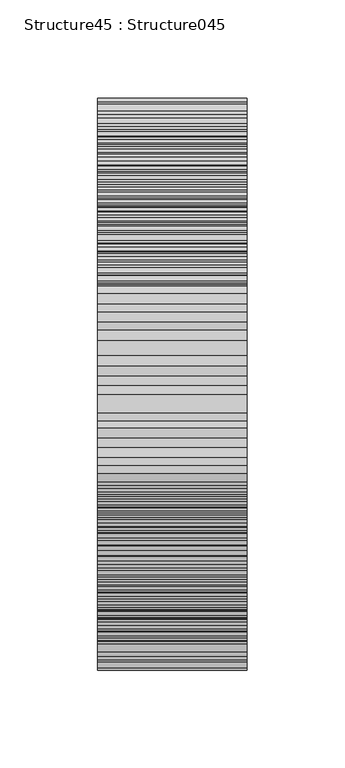
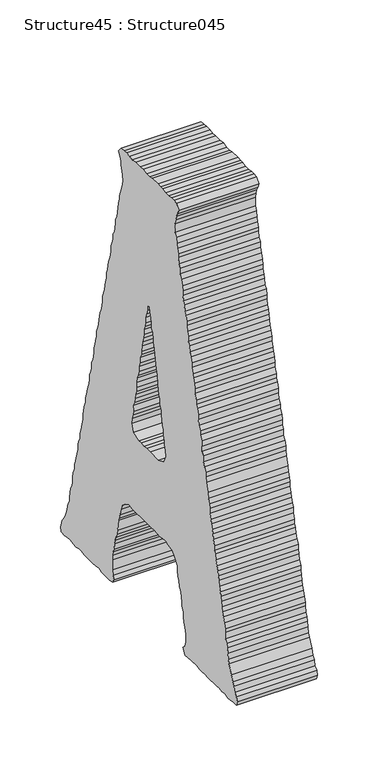
"""IFC4 building model written with IfcOpenShell, lengths in millimetres: proxy geometry, Structure45 : Structure045."""

from ifc_helpers import new_model, si_unit, frame, origin, place, context, project, spatial, polyline, outline, extrude, source, transform, mapped, element, save


def structure45_structure045_837fe079(model_context):
    return source(origin(), model_context, "Body", "SweptSolid", [
        extrude(outline(polyline([(253886.5092101, 3818.8310229), (253888.8599557, 3824.1149855), (253889.4440317, 3828.2163546), (253890.0281078, 3833.4730389), (253891.7947773, 3838.1761347), (253892.3772487, 3841.6741725), (253894.1262676, 3846.9757858), (253894.1262676, 3851.6612309), (253895.8929372, 3856.9179152), (253897.0610893, 3861.0192843), (253898.2260321, 3866.3032469), (253899.4118349, 3870.4030114), (253899.9943063, 3875.0772243), (253901.7433252, 3878.5784713), (253902.3354242, 3884.4609514), (253902.3354242, 3888.5623205), (253903.5099947, 3893.822214), (253905.2622228, 3896.763454), (253906.4367933, 3902.6314927), (253907.6113638, 3906.1487857), (253908.7795159, 3910.8310217), (253908.7795159, 3915.5068392), (253909.9540864, 3919.6066036), (253911.7031053, 3924.8905662), (253913.4617518, 3929.5904528), (253913.4617518, 3934.8503464), (253915.2203983, 3938.3499888), (253916.3965734, 3944.235678), (253916.3965734, 3947.7337158), (253918.15522, 3952.435207), (253918.7457144, 3957.1190475), (253919.9138665, 3962.3757319), (253921.6709084, 3966.5043792), (253921.6709084, 3974.7055128), (253920.4947333, 3979.3781211), (253919.3201628, 3984.0635662), (253917.5711439, 3987.5792547), (253915.2203983, 3992.2614906), (253919.3201628, 3996.9645864), (253923.4215319, 3997.5486624), (253927.530924, 3997.5486624), (253932.805259, 3996.390138), (253937.4874949, 3996.390138), (253942.7650391, 3997.5486624), (253946.2727045, 3996.9645864), (253950.3837013, 3997.5486624), (253959.7594053, 3997.5486624), (253964.4320136, 3996.390138), (253969.1254818, 3996.390138), (253974.4094444, 3997.5486624), (253979.6677333, 3996.9645864), (253987.2847908, 3996.9645864), (253992.5687535, 3996.390138), (253996.6685179, 3997.5486624), (254001.9348299, 3997.5486624), (254006.036199, 3996.9645864), (254011.310534, 3996.390138), (254014.8294316, 3991.6806238), (254012.4963367, 3987.5792547), (254011.310534, 3983.4794902), (254010.7296671, 3979.9621971), (254009.553492, 3974.7055128), (254007.8028685, 3965.8930249), (254008.9806482, 3961.794865), (254010.1359635, 3956.5349715), (254013.6532565, 3947.1496398), (254013.6532565, 3944.235678), (254014.8294316, 3938.9517154), (254016.0040021, 3934.2758979), (254016.5880781, 3928.9919353), (254017.7546256, 3924.2888396), (254020.1133942, 3919.6066036), (254020.1133942, 3916.0909152), (254020.6894472, 3910.8310217), (254021.8640177, 3906.1487857), (254024.2051357, 3902.6314927), (254024.2051357, 3897.3475301), (254025.9637822, 3892.6636896), (254027.1383527, 3888.5623205), (254027.1383527, 3883.8881076), (254028.3049002, 3878.5784713), (254030.0651513, 3873.9203044), (254031.8237978, 3869.8189354), (254032.4046647, 3866.3032469), (254032.9983683, 3861.0192843), (254034.7554102, 3856.9179152), (254034.7554102, 3851.6612309), (254036.5060338, 3846.9757858), (254037.0981328, 3842.8583706), (254038.2727033, 3837.6000817), (254041.1995019, 3829.374879), (254041.1995019, 3824.1149855), (254042.3740724, 3820.015221), (254043.5390153, 3815.3313805), (254045.8897608, 3810.0474179), (254046.4738369, 3806.5317294), (254047.6403843, 3801.8462843), (254048.2324834, 3797.1463977), (254049.9911299, 3791.8865042), (254051.1560728, 3788.3611881), (254051.1560728, 3783.0868532), (254052.9147193, 3777.8285642), (254053.508423, 3774.3032481), (254055.2574419, 3769.0176809), (254055.8495409, 3764.3611187), (254056.433617, 3759.6596275), (254057.6081875, 3756.1423345), (254059.3572064, 3751.4424479), (254059.95091, 3745.6000829), (254061.1254805, 3740.9162424), (254062.8744994, 3737.9750024), (254062.8744994, 3732.7167134), (254064.0506745, 3727.4311462), (254065.801298, 3723.3313817), (254066.9758685, 3718.0554422), (254068.150439, 3714.5301261), (254069.3169865, 3710.4560353), (254069.3169865, 3705.7545441), (254071.6693367, 3699.8881101), (254072.8342795, 3695.2122926), (254073.4183556, 3691.0868544), (254073.4183556, 3686.4030139), (254074.5929261, 3682.8857208), (254076.3595956, 3677.0449604), (254076.9356486, 3673.5276674), (254078.7023182, 3668.8261762), (254078.7023182, 3663.5598643), (254081.0354131, 3659.4584952), (254082.2099836, 3655.3587307), (254082.2099836, 3650.6845178), (254083.3845541, 3645.4262289), (254085.133573, 3640.114988), (254086.3193757, 3636.0408972), (254087.4859232, 3632.5155811), (254088.0683946, 3627.2396415), (254089.8270411, 3622.555801), (254091.0016116, 3617.2718384), (254091.0016116, 3612.5976255), (254091.5776646, 3608.4705827), (254093.9364333, 3604.3964919), (254095.1029807, 3599.1125293), (254096.2711328, 3594.4286888), (254096.2711328, 3590.3289243), (254098.0378023, 3586.2115092), (254100.9613917, 3576.2693797), (254102.7104106, 3572.1423369), (254104.4786848, 3568.6426945), (254107.9863502, 3563.366755), (254109.1721529, 3560.441561), (254110.9211718, 3555.1848766), (254109.7530198, 3551.0658569), (254103.8881903, 3550.4833855), (254100.3692927, 3551.0658569), (254095.1029807, 3551.6675836), (254090.4207448, 3550.4833855), (254085.133573, 3550.4833855), (254080.4513371, 3551.6675836), (254076.3595956, 3551.6675836), (254071.6693367, 3551.0658569), (254067.5679676, 3551.0658569), (254061.6999289, 3550.4833855), (254057.6081875, 3550.4833855), (254052.9147193, 3551.0658569), (254047.6403843, 3551.6675836), (254043.5390153, 3550.4833855), (254030.0651513, 3550.4833855), (254024.7876071, 3551.6675836), (254022.4480938, 3555.7416744), (254024.2051357, 3559.2669905), (254025.3797062, 3563.9412034), (254025.3797062, 3573.9266571), (254025.3797062, 3578.6104977), (254024.2051357, 3582.7102621), (254022.4480938, 3586.2115092), (254021.8640177, 3592.0955938), (254020.6894472, 3596.1953583), (254018.9291961, 3600.2967274), (254017.7546256, 3604.3964919), (254016.5880781, 3609.0723094), (254015.4199261, 3619.6145609), (254014.2469602, 3622.555801), (254012.4963367, 3627.2396415), (254011.310534, 3633.0980525), (254008.3869446, 3638.9580681), (254004.2871801, 3642.4833842), (253997.83667, 3645.9830266), (253993.1528295, 3644.8245022), (253983.7771254, 3644.8245022), (253977.9171098, 3645.4262289), (253965.6178163, 3645.4262289), (253960.3322491, 3644.8245022), (253956.2421123, 3645.9830266), (253951.5566671, 3645.4262289), (253946.8664082, 3644.8245022), (253942.7650391, 3645.4262289), (253936.9066281, 3645.9830266), (253933.389335, 3644.8245022), (253926.362772, 3643.0578326), (253922.8374559, 3639.5405396), (253918.15522, 3633.0980525), (253918.15522, 3627.8397636), (253916.9774403, 3622.555801), (253915.2203983, 3619.6145609), (253914.6443453, 3613.772196), (253912.2952043, 3610.2292293), (253911.1286569, 3604.9709403), (253910.5381624, 3601.4536473), (253910.5381624, 3596.7698067), (253908.1858122, 3592.0955938), (253907.6113638, 3587.3860796), (253907.0288924, 3582.7102621), (253905.2622228, 3578.6104977), (253903.5099947, 3572.7440636), (253904.0860477, 3565.1254015), (253905.8446943, 3559.2669905), (253908.7795159, 3556.3417965), (253905.2622228, 3550.4833855), (253899.9943063, 3551.0658569), (253895.3024427, 3551.6675836), (253885.9267387, 3551.6675836), (253881.2428981, 3551.0658569), (253876.5606622, 3551.0658569), (253872.4496655, 3551.6675836), (253868.349901, 3551.0658569), (253862.49149, 3551.0658569), (253858.98222, 3551.6675836), (253853.1141813, 3551.0658569), (253849.5984929, 3551.6675836), (253844.9066293, 3550.4833855), (253839.6387128, 3551.6675836), (253834.3627732, 3550.4833855), (253830.2630087, 3551.0658569), (253825.5711452, 3551.6675836), (253820.8953277, 3551.6675836), (253819.1286581, 3556.3417965), (253820.3032286, 3560.441561), (253823.2380502, 3563.366755), (253824.4029931, 3568.6426945), (253826.1616396, 3572.1423369), (253828.5139898, 3577.4535778), (253832.6137543, 3586.2115092), (253833.7786972, 3589.7544759), (253834.3627732, 3595.5872132), (253835.5373437, 3600.2967274), (253836.7054958, 3604.3964919), (253838.4721653, 3607.8961343), (253839.0562414, 3613.772196), (253839.0562414, 3617.2718384), (253840.2227888, 3622.555801), (253841.9814353, 3627.8397636), (253843.7481049, 3631.915459), (253844.9066293, 3636.0408972), (253845.4971238, 3641.2991861), (253846.0908275, 3645.9830266), (253846.6716943, 3650.1004418), (253849.0144169, 3654.1841602), (253849.5984929, 3660.0682449), (253850.1905919, 3664.1423357), (253850.7730634, 3668.8261762), (253852.5220823, 3672.9435914), (253854.2887518, 3677.6274319), (253855.4569039, 3682.8857208), (253856.6314744, 3685.8285655), (253856.6314744, 3690.512406), (253858.3901209, 3695.786741), (253858.98222, 3701.0723082), (253860.1391398, 3704.5879966), (253861.907414, 3709.2718371), (253862.49149, 3713.3555556), (253864.2485319, 3718.6571688), (253864.2485319, 3723.3313817), (253865.4263116, 3727.4311462), (253866.5912545, 3732.1149867), (253867.7561974, 3737.400554), (253870.1085476, 3746.1745313), (253871.2766996, 3750.8583719), (253871.2766996, 3755.559863), (253873.0433692, 3759.6596275), (253874.7923881, 3763.759392), (253874.7923881, 3769.6274306), (253877.1415291, 3773.11905), (253877.1415291, 3777.8285642), (253877.7159775, 3783.0868532), (253880.0683277, 3787.7867397), (253880.0683277, 3791.8865042), (253882.4094456, 3795.960595), (253882.991917, 3801.8462843), (253882.991917, 3805.9476534), (253885.3346396, 3811.2043377), (253886.5092101, 3814.7296538), (253886.5092101, 3818.8310229)]), holes=[polyline([(253949.1978985, 3720.4158154), (253962.6829947, 3720.4158154), (253967.9493067, 3720.9726131), (253973.2348739, 3719.8140887), (253977.3330338, 3720.9726131), (253981.4344029, 3720.4158154), (253990.2196125, 3723.3313817), (253993.1528295, 3730.9323932), (253991.978259, 3736.7988273), (253990.8004793, 3740.9162424), (253989.6451641, 3744.9999608), (253990.2196125, 3750.8583719), (253987.8768899, 3754.9854146), (253987.2847908, 3759.6596275), (253986.7023194, 3763.759392), (253984.9516959, 3767.8607611), (253984.3612015, 3772.5606477), (253984.3612015, 3777.2444882), (253983.7771254, 3782.5027771), (253982.0265019, 3786.0280932), (253980.8519314, 3790.7039107), (253980.8519314, 3795.4037973), (253978.5108135, 3800.6717138), (253978.5108135, 3805.9476534), (253976.7425393, 3810.0474179), (253976.1584633, 3813.5743386), (253975.5663642, 3819.4150989), (253974.4094444, 3824.1149855), (253973.2348739, 3828.790803), (253972.6427748, 3832.8921721), (253972.6427748, 3837.6000817), (253970.3000523, 3842.2758992), (253969.7159762, 3846.3772683), (253969.7159762, 3851.6612309), (253967.9493067, 3856.3161885), (253966.7923868, 3860.4432313), (253966.7923868, 3864.5446004), (253965.0257173, 3865.1190488), (253963.8591698, 3860.4432313), (253962.0989187, 3855.7353217), (253961.5084242, 3851.0595042), (253961.5084242, 3845.8012153), (253959.1753293, 3842.2758992), (253958.5816256, 3836.9919366), (253958.5816256, 3833.4730389), (253956.2421123, 3828.790803), (253955.6580362, 3822.932392), (253955.0659372, 3818.8310229), (253953.8913667, 3814.7296538), (253953.3072907, 3810.0474179), (253951.5566671, 3804.7730829), (253950.9645681, 3795.4037973), (253949.7899976, 3790.7039107), (253949.1978985, 3786.0280932), (253947.447275, 3783.0868532), (253947.447275, 3777.8285642), (253945.1061571, 3773.11905), (253945.1061571, 3768.4432325), (253943.9315866, 3764.3611187), (253943.3475105, 3759.0595054), (253941.5792364, 3755.559863), (253941.5792364, 3750.3015741), (253939.8302175, 3744.9999608), (253939.8302175, 3741.5003184), (253938.655647, 3736.7988273), (253937.4874949, 3730.9323932), (253941.0063926, 3723.9154578), (253949.1978985, 3720.4158154)])]), frame((-38594.2176606, 0.0, 0.0), z_axis=(1.0, 0.0, 0.0), x_axis=(0.0, 1.0, 0.0)), (0.0, 0.0, 1.0), 76.2),
    ])


if __name__ == "__main__":
    model = new_model("IFC4")
    model_context = context("Model", 3, world=origin())
    ifc_project = project(units=[si_unit("LENGTHUNIT", "METRE", prefix="MILLI")], contexts=[model_context])
    site = spatial("IfcSite", under=ifc_project)
    building = spatial("IfcBuilding", under=site)
    placement = place(None, origin())
    structure45_structure045_shape = structure45_structure045_837fe079(model_context)
    element("IfcBuildingElementProxy", 1, Name="Structure45 : Structure045", ObjectType="Structure45 : Structure045", at=placement, inside=building, context=model_context, shape_type="MappedRepresentation", body=[
        mapped(structure45_structure045_shape, transform((0.0, 0.0, 0.0), x_axis=(1.0, 0.0, 0.0), y_axis=(0.0, 1.0, 0.0), z_axis=(0.0, 0.0, 1.0))),
    ])
    save(model, "model.ifc")

# Revit data of these elements
# Type "Structure45 : Structure045"
#   NameOverride = "Structure045"
# Element 1 (IfcBuildingElementProxy, "Structure45 : Structure045")
#   Materials on its faces: "BRUSHED ALUM. LETTERING"
# Materials
#   "BRUSHED ALUM. LETTERING": class "Unassigned", colour RGB 169 181 186, transparency 0, Cost = 0
